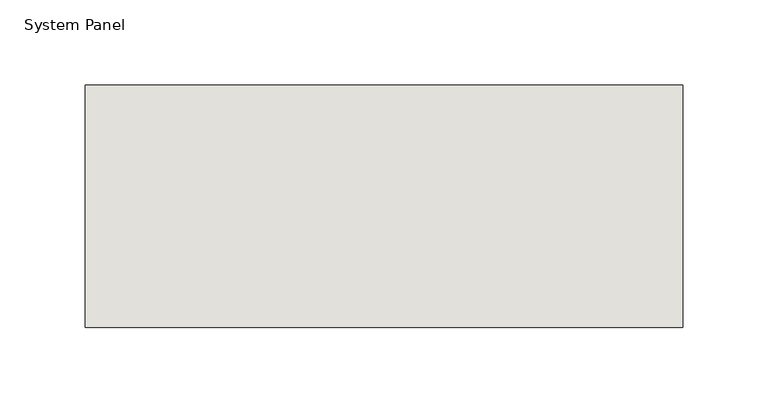
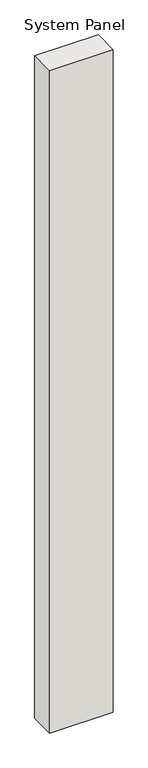
"""IFC4 building model written with IfcOpenShell, lengths in millimetres: wall geometry, System Panel : NLRS_21_CWP_hsb-vulling minerale wol 142 _gen_rsf."""

from ifc_helpers import new_model, si_unit, origin, origin_with_axes, place, context, project, spatial, polyline, outline, extrude, source, transform, mapped, element, save


def system_panel_cc2e8257(model_context):
    return source(origin(), model_context, "Body", "SweptSolid", [
        extrude(outline(polyline([(175.0000002, -71.0), (-175.0000002, -71.0), (-175.0000002, 71.0), (175.0000002, 71.0), (175.0000002, -71.0)])), origin_with_axes(), (0.0, 0.0, 1.0), 3849.0),
    ])


if __name__ == "__main__":
    model = new_model("IFC4")
    model_context = context("Model", 3, world=origin())
    ifc_project = project(units=[si_unit("LENGTHUNIT", "METRE", prefix="MILLI")], contexts=[model_context])
    site = spatial("IfcSite", under=ifc_project)
    building = spatial("IfcBuilding", under=site)
    placement = place(None, origin())
    system_panel_shape = system_panel_cc2e8257(model_context)
    element("IfcWall", 1, ObjectType="System Panel : NLRS_21_CWP_hsb-vulling minerale wol 142 _gen_rsf", at=placement, inside=building, context=model_context, shape_type="MappedRepresentation", body=[
        mapped(system_panel_shape, transform((0.0, 0.0, 0.0), x_axis=(1.0, 0.0, 0.0), y_axis=(0.0, 1.0, 0.0), z_axis=(0.0, 0.0, 1.0))),
    ])
    save(model, "model.ifc")

# Revit data of these elements
# Type "System Panel : NLRS_21_CWP_hsb-vulling minerale wol 142 _gen_rsf"
#   Type IfcGUID = "07M7mRoiH1CR8m_RSKIwpC"
#   Assembly Code = "21.23"
#   IfcExportAs = "IfcWall"
# Element 1 (IfcWall, "System Panel : NLRS_21_CWP_hsb-vulling minerale wol 142 _gen_rsf")
#   Materials on its faces: "NLRS_m1_isolatie minerale wol_gen_rsf"
# Materials
#   "NLRS_m1_isolatie minerale wol_gen_rsf": class "M - Anorganische materialen", colour RGB 200 200 140, transparency 0, Keynote = "m1", Manufacturer = "Revit Standards Foundation", URL = "www.revitstandards.org", Description = "isolatie minerale wol", Cost = 0
